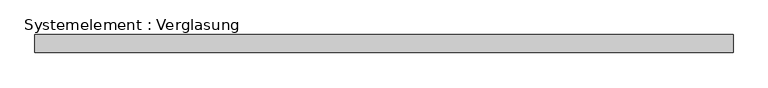
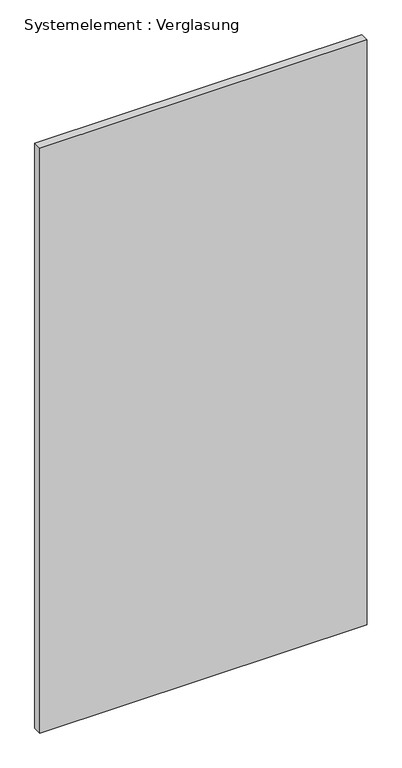
"""IFC4 building model written with IfcOpenShell, lengths in millimetres: plate geometry, Systemelement : Verglasung."""

from ifc_helpers import new_model, si_unit, origin, origin_with_axes, place, context, project, spatial, polyline, outline, extrude, source, transform, mapped, element, save


def systemelement_verglasung_7f313b09(model_context):
    return source(origin(), model_context, "Body", "SweptSolid", [
        extrude(outline(polyline([(580.0000002, -15.0), (-580.0000002, -15.0), (-580.0000002, 15.0), (580.0000002, 15.0), (580.0000002, -15.0)])), origin_with_axes(), (0.0, 0.0, 1.0), 2190.0),
    ])


if __name__ == "__main__":
    model = new_model("IFC4")
    model_context = context("Model", 3, world=origin())
    ifc_project = project(units=[si_unit("LENGTHUNIT", "METRE", prefix="MILLI")], contexts=[model_context])
    site = spatial("IfcSite", under=ifc_project)
    building = spatial("IfcBuilding", under=site)
    placement = place(None, origin())
    systemelement_verglasung_shape = systemelement_verglasung_7f313b09(model_context)
    element("IfcPlate", 1, ObjectType="Systemelement : Verglasung", at=placement, inside=building, context=model_context, shape_type="MappedRepresentation", body=[
        mapped(systemelement_verglasung_shape, transform((0.0, 0.0, 0.0), x_axis=(1.0, 0.0, 0.0), y_axis=(0.0, 1.0, 0.0), z_axis=(0.0, 0.0, 1.0))),
    ])
    save(model, "model.ifc")

# Revit data of these elements
# Type "Systemelement : Verglasung"
#   Construction Type Id = "GSP4R"
#   Analytic Construction = "1/8 Zoll Pilkington-Verglasung einfach"
#   Visual Light Transmittance = 0.9
#   Solar Heat Gain Coefficient = 0.86
#   Heat Transfer Coefficient (U) = 6.7069 W/(m²·K)
# Element 1 (IfcPlate, "Systemelement : Verglasung")
#   Materials on its faces: "Glas"
# Materials
#   "Glas": class "Glas", colour RGB 0 0 255, transparency 0.75, Comments = "Render-Darstellung nicht aktualisiert ", Cost = 0
